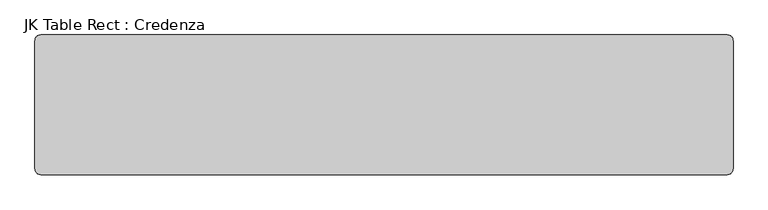
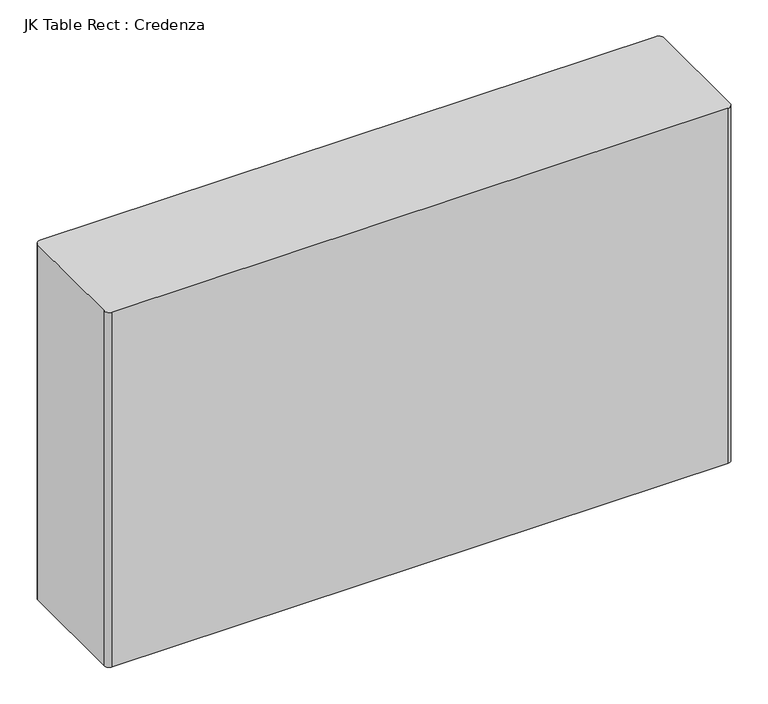
"""IFC4 building model written with IfcOpenShell, lengths in millimetres: furniture geometry, JK Table Rect : Credenza."""

from ifc_helpers import new_model, si_unit, point, frame_2d, origin, origin_with_axes, place, context, project, spatial, polyline, circle_curve, trimmed, segment, composite_curve, outline, extrude, source, transform, mapped, element, save


def jk_table_rect_credenza_90bb0585(model_context):
    return source(origin(), model_context, "Body", "SweptSolid", [
        extrude(outline(composite_curve([segment(polyline([(687.3573665, -185.9455296), (-811.2426335, -185.9455296)]), True, "CONTINUOUS"), segment(trimmed(circle_curve(frame_2d((-811.2426335, -173.2455296)), 12.7), [point((-811.2426335, -185.9455296))], [point((-823.9426335, -173.2455296))], False, "CARTESIAN"), True, "CONTINUOUS"), segment(polyline([(-823.9426335, -173.2455296), (-823.9426335, 106.1544704)]), True, "CONTINUOUS"), segment(trimmed(circle_curve(frame_2d((-811.2426335, 106.1544704)), 12.7), [point((-823.9426335, 106.1544704))], [point((-811.2426335, 118.8544704))], False, "CARTESIAN"), True, "CONTINUOUS"), segment(polyline([(-811.2426335, 118.8544704), (687.3573665, 118.8544704)]), True, "CONTINUOUS"), segment(trimmed(circle_curve(frame_2d((687.3573665, 106.1544704)), 12.7), [point((687.3573665, 118.8544704))], [point((700.0573665, 106.1544704))], False, "CARTESIAN"), True, "CONTINUOUS"), segment(polyline([(700.0573665, 106.1544704), (700.0573665, -173.2455296)]), True, "CONTINUOUS"), segment(trimmed(circle_curve(frame_2d((687.3573665, -173.2455296)), 12.7), [point((700.0573665, -173.2455296))], [point((687.3573665, -185.9455296))], False, "CARTESIAN"), True, "CONTINUOUS")], self_intersect=False)), origin_with_axes(), (0.0, 0.0, 1.0), 914.4),
    ])


if __name__ == "__main__":
    model = new_model("IFC4")
    model_context = context("Model", 3, world=origin())
    ifc_project = project(units=[si_unit("LENGTHUNIT", "METRE", prefix="MILLI")], contexts=[model_context])
    site = spatial("IfcSite", under=ifc_project)
    building = spatial("IfcBuilding", under=site)
    placement = place(None, origin())
    jk_table_rect_credenza_shape = jk_table_rect_credenza_90bb0585(model_context)
    element("IfcFurniture", 1, ObjectType="JK Table Rect : Credenza", at=placement, inside=building, context=model_context, shape_type="MappedRepresentation", body=[
        mapped(jk_table_rect_credenza_shape, transform((0.0, 0.0, 0.0), x_axis=(1.0, 0.0, 0.0), y_axis=(0.0, 1.0, 0.0), z_axis=(0.0, 0.0, 1.0))),
    ])
    save(model, "model.ifc")

# Revit data of these elements
# Type "JK Table Rect : Credenza"
#   Width = 5' - 0"
#   Height = 3' - 0"
#   Depth = 1' - 0"
#   Corner Radius = 0' - 0 1/2"
#   Status [instance default] = none
#   Default Elevation = 0
